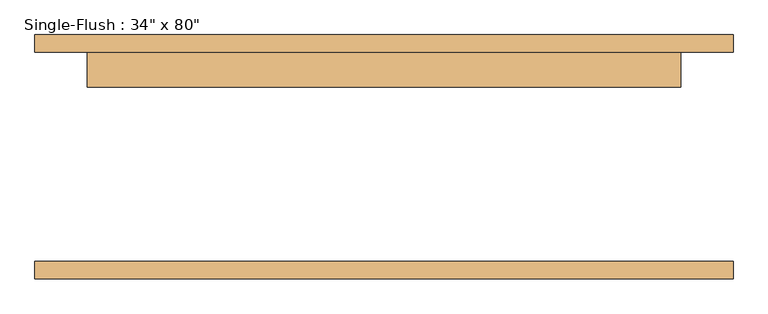
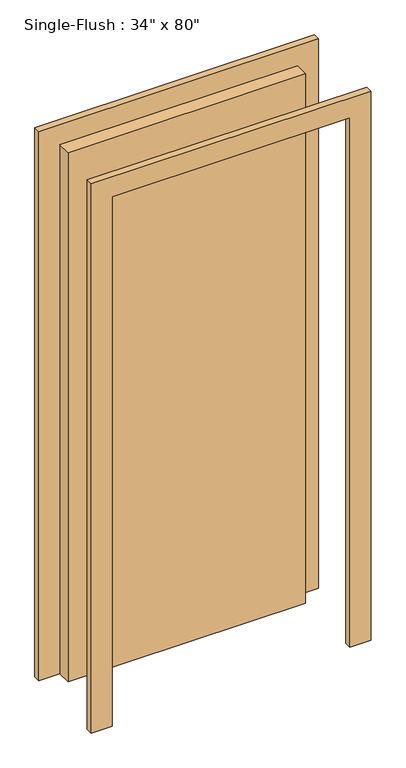
"""IFC4 building model written with IfcOpenShell, lengths in millimetres: door geometry."""

import ifcopenshell
import ifcopenshell.guid

model = None  # the IFC model being written
_history = None  # IfcOwnerHistory: only IFC2X3 demands one
_inside = {}  # id of a spatial element -> (the spatial element, [elements in it])
_under = {}  # id of a project, library or spatial element -> (it, [spatial elements below it])
_declared = {}  # id of a project -> (the project, [libraries it declares])
_typed = {}  # id of a type object -> (the type object, [elements of that type])
_made_of = {}  # id of a material, layer set ... -> (it, [elements and type objects made of it])


def new_model(schema):
    """Start an empty IFC model of exactly this schema.

    Asked for "IFC4X3", IfcOpenShell would pick the latest addendum, in which some entities
    have other attributes; the version numbers below select the first issue.
    IFC2X3 requires an IfcOwnerHistory on every rooted entity: one is made here for all.
    """
    global model, _history
    if schema == "IFC4X3":
        model = ifcopenshell.file(schema_version=(4, 3, 0, 0))
    else:
        model = ifcopenshell.file(schema=schema)
    _inside.clear()
    _under.clear()
    _declared.clear()
    _typed.clear()
    _made_of.clear()
    _history = None
    if model.schema == "IFC2X3":
        org = make("IfcOrganization", Name="unknown")
        user = make(
            "IfcPersonAndOrganization",
            ThePerson=make("IfcPerson", FamilyName="unknown"),
            TheOrganization=org,
        )
        app = make(
            "IfcApplication",
            ApplicationDeveloper=org,
            Version="unknown",
            ApplicationFullName="unknown",
            ApplicationIdentifier="unknown",
        )
        _history = make(
            "IfcOwnerHistory",
            OwningUser=user,
            OwningApplication=app,
            ChangeAction="ADDED",
            CreationDate=0,
        )
    return model


def make(cls, **values):
    """One entity of the class cls with the attributes given. An attribute that is None is left unset."""
    return model.create_entity(
        cls, **{name: value for name, value in values.items() if value is not None}
    )


def rooted(cls, **values):
    """An entity with a GlobalId (a new one), such as an element, a storey or a relation."""
    return make(cls, GlobalId=ifcopenshell.guid.new(), OwnerHistory=_history, **values)


def si_unit(unit_type, name, prefix=None):
    """IfcSIUnit, for example si_unit("LENGTHUNIT", "METRE", prefix="MILLI")."""
    return make("IfcSIUnit", UnitType=unit_type, Prefix=prefix, Name=name)


def assignment(units):
    """IfcUnitAssignment: the units of a project."""
    return None if units is None else make("IfcUnitAssignment", Units=units)


def point(xyz):
    """IfcCartesianPoint."""
    return None if xyz is None else make("IfcCartesianPoint", Coordinates=xyz)


def direction(xyz):
    """IfcDirection."""
    return None if xyz is None else make("IfcDirection", DirectionRatios=xyz)


def frame(location, z_axis=None, x_axis=None):
    """IfcAxis2Placement3D, a coordinate frame: its origin and axes. An axis left out is left unset."""
    return make(
        "IfcAxis2Placement3D",
        Location=point(location),
        Axis=direction(z_axis),
        RefDirection=direction(x_axis),
    )


def origin():
    """The frame at (0, 0, 0) with its axes left unset."""
    return frame((0.0, 0.0, 0.0))


def origin_with_axes():
    """The frame at (0, 0, 0) with the z axis (0, 0, 1) and the x axis (1, 0, 0) written out."""
    return frame((0.0, 0.0, 0.0), z_axis=(0.0, 0.0, 1.0), x_axis=(1.0, 0.0, 0.0))


def place(relative_to, where):
    """IfcLocalPlacement: puts the frame where relative to a parent placement (None: the world)."""
    return make(
        "IfcLocalPlacement", PlacementRelTo=relative_to, RelativePlacement=where
    )


def context(
    kind, dimensions, precision=None, world=None, true_north=None, identifier=None
):
    """IfcGeometricRepresentationContext, for example the 3D "Model" context."""
    return make(
        "IfcGeometricRepresentationContext",
        ContextIdentifier=identifier,
        ContextType=kind,
        CoordinateSpaceDimension=dimensions,
        Precision=precision,
        WorldCoordinateSystem=world,
        TrueNorth=true_north,
    )


def project(units=None, contexts=None):
    """IfcProject with its units and contexts."""
    return rooted(
        "IfcProject",
        Name="project",
        RepresentationContexts=contexts,
        UnitsInContext=assignment(units),
    )


def spatial(cls, under=None, at=None, **own):
    """A site, building, storey or space (cls), placed at a placement, below another one or the project."""
    s = rooted(cls, ObjectPlacement=at, **own)
    if under is not None:
        _under.setdefault(under.id(), (under, []))[1].append(s)
    return s


def polyline(points):
    """IfcPolyline through the points."""
    return make("IfcPolyline", Points=[point(p) for p in points])


def outline(outer, holes=None, kind="AREA"):
    """IfcArbitraryClosedProfileDef: a profile drawn as a closed curve; with holes, ...WithVoids."""
    if holes is None:
        return make("IfcArbitraryClosedProfileDef", ProfileType=kind, OuterCurve=outer)
    return make(
        "IfcArbitraryProfileDefWithVoids",
        ProfileType=kind,
        OuterCurve=outer,
        InnerCurves=holes,
    )


def extrude(swept, where, along, depth):
    """IfcExtrudedAreaSolid: the profile swept, set in the frame where, extruded along a direction by depth."""
    return make(
        "IfcExtrudedAreaSolid",
        SweptArea=swept,
        Position=where,
        ExtrudedDirection=direction(along),
        Depth=depth,
    )


def shape(context_of_items, identifier, shape_type, items):
    """IfcShapeRepresentation: the items that make up one representation, for example the "Body"."""
    return make(
        "IfcShapeRepresentation",
        ContextOfItems=context_of_items,
        RepresentationIdentifier=identifier,
        RepresentationType=shape_type,
        Items=items,
    )


def source(mapping_origin, context_of_items, identifier, shape_type, items):
    """IfcRepresentationMap: a shape defined once, which mapped items show again and again."""
    return make(
        "IfcRepresentationMap",
        MappingOrigin=mapping_origin,
        MappedRepresentation=shape(context_of_items, identifier, shape_type, items),
    )


def transform(
    local_origin,
    x_axis=None,
    y_axis=None,
    z_axis=None,
    scale=None,
    scale2=None,
    scale3=None,
    uniform=True,
):
    """IfcCartesianTransformationOperator3D, or its non-uniform kind. x_axis, y_axis, z_axis: its Axis1, 2, 3."""
    if uniform:
        return make(
            "IfcCartesianTransformationOperator3D",
            Axis1=direction(x_axis),
            Axis2=direction(y_axis),
            LocalOrigin=point(local_origin),
            Scale=scale,
            Axis3=direction(z_axis),
        )
    return make(
        "IfcCartesianTransformationOperator3DnonUniform",
        Axis1=direction(x_axis),
        Axis2=direction(y_axis),
        LocalOrigin=point(local_origin),
        Scale=scale,
        Axis3=direction(z_axis),
        Scale2=scale2,
        Scale3=scale3,
    )


def mapped(mapping_source, mapping_target):
    """IfcMappedItem: shows the shape of a source again, moved by a transform."""
    return make(
        "IfcMappedItem", MappingSource=mapping_source, MappingTarget=mapping_target
    )


def made_of(thing, what):
    """Note that an element or type object is made of a material, layer set ...; save() writes the relation."""
    if what is not None:
        _made_of.setdefault(what.id(), (what, []))[1].append(thing)
    return thing


def element(
    cls,
    number,
    at=None,
    inside=None,
    cuts=None,
    type_object=None,
    material=None,
    context=None,
    identifier="Body",
    shape_type=None,
    held_by="IfcProductDefinitionShape",
    body=None,
    shapes=None,
    **own,
):
    """One element of the class cls, such as IfcWall. Its Tag is "e" and its number.

    at: its placement. inside: the storey or other place that contains it. cuts: it is an
    opening in that element (IfcRelVoidsElement). A single representation is given by context,
    identifier, shape_type and body (its items); several are given by shapes. held_by: the class
    of the entity that holds the representations. save() writes the other relations.
    """
    e = rooted(cls, Tag="e%d" % number, ObjectPlacement=at, **own)
    if body is not None:
        shapes = [shape(context, identifier, shape_type, body)]
    if shapes is not None:
        e.Representation = make(held_by, Representations=shapes)
    if inside is not None:
        _inside.setdefault(inside.id(), (inside, []))[1].append(e)
    if cuts is not None:
        rooted(
            "IfcRelVoidsElement", RelatingBuildingElement=cuts, RelatedOpeningElement=e
        )
    if type_object is not None:
        _typed.setdefault(type_object.id(), (type_object, []))[1].append(e)
    return made_of(e, material)


def aggregate(whole, parts):
    """IfcRelAggregates: a whole, such as a stair, and the parts it consists of."""
    return rooted("IfcRelAggregates", RelatingObject=whole, RelatedObjects=parts)


def save(model, path):
    """Write the relations noted so far, then the file.

    IfcRelAggregates (storeys below a building ...), IfcRelContainedInSpatialStructure (elements
    in a storey), IfcRelDefinesByType, IfcRelAssociatesMaterial and IfcRelDeclares: one each for
    every whole, place, type object, material and project.
    """
    for whole, parts in _under.values():
        aggregate(whole, parts)
    for where, things in _inside.values():
        rooted(
            "IfcRelContainedInSpatialStructure",
            RelatedElements=things,
            RelatingStructure=where,
        )
    for kind, things in _typed.values():
        rooted("IfcRelDefinesByType", RelatedObjects=things, RelatingType=kind)
    for what, things in _made_of.values():
        rooted("IfcRelAssociatesMaterial", RelatedObjects=things, RelatingMaterial=what)
    for by, libraries in _declared.values():
        rooted("IfcRelDeclares", RelatingContext=by, RelatedDefinitions=libraries)
    model.write(path)


def door_93553381(model_context):
    return source(origin(), model_context, "Body", "SweptSolid", [
        extrude(outline(polyline([(2108.2, -508.0), (0.0, -508.0), (0.0, -431.8), (2032.0, -431.8), (2032.0, 431.8), (0.0, 431.8), (0.0, 508.0), (2108.2, 508.0), (2108.2, -508.0)])), frame((0.0, 152.4, 0.0), z_axis=(0.0, 1.0, 0.0), x_axis=(0.0, 0.0, 1.0)), (0.0, 0.0, 1.0), 25.4),
        extrude(outline(polyline([(2108.2, 508.0), (2108.2, -508.0), (0.0, -508.0), (0.0, -431.8), (2032.0, -431.8), (2032.0, 431.8), (0.0, 431.8), (0.0, 508.0), (2108.2, 508.0)])), frame((0.0, -177.8, 0.0), z_axis=(0.0, 1.0, 0.0), x_axis=(0.0, 0.0, 1.0)), (0.0, 0.0, 1.0), 25.4),
        extrude(outline(polyline([(431.8, 101.6), (-431.8, 101.6), (-431.8, 152.4), (431.8, 152.4), (431.8, 101.6)])), origin_with_axes(), (0.0, 0.0, 1.0), 2032.0),
    ])


if __name__ == "__main__":
    model = new_model("IFC4")
    model_context = context("Model", 3, world=origin())
    ifc_project = project(units=[si_unit("LENGTHUNIT", "METRE", prefix="MILLI")], contexts=[model_context])
    site = spatial("IfcSite", under=ifc_project)
    building = spatial("IfcBuilding", under=site)
    placement = place(None, origin())
    door_shape = door_93553381(model_context)
    element("IfcDoor", 1, ObjectType="Single-Flush : 34\" x 80\"", at=placement, inside=building, context=model_context, shape_type="MappedRepresentation", body=[
        mapped(door_shape, transform((0.0, 0.0, 0.0), x_axis=(1.0, 0.0, 0.0), y_axis=(0.0, 1.0, 0.0), z_axis=(0.0, 0.0, 1.0))),
    ])
    save(model, "model.ifc")

# Revit data of these elements
# Type "Single-Flush : 34\" x 80\""
#   Type Mark = "7"
#   Construction Type Id = "MDOOR"
#   Assembly Code = "C1020"
#   Analytic Construction = "Metal"
#   Thickness = 0' - 2"
#   Heat Transfer Coefficient (U) = 0.651978 BTU/(h·ft²·°F)
#   Height = 6' - 8"
#   Trim Projection Ext = 0' - 1"
#   Trim Projection Int = 0' - 1"
#   Trim Width = 0' - 3"
#   Width = 2' - 10"
#   Define Thermal Properties by = 1
#   Define Thermal Properties by = 1
#   Door Material = Door - Panel
#   Frame Material = Door - Frame
#   Visual Light Transmittance = 0
#   Solar Heat Gain Coefficient = 0
#   Function = (empty or 0)
#   Wall Closure = (empty or 0)
# Element 1 (IfcDoor, "Single-Flush : 34\" x 80\"")
#   Materials on its faces: "Door - Frame", "Door - Panel"
# Materials
#   "Door - Panel": class "Wood", colour RGB 210 159 95, transparency 0, Cost = 0
#   "Door - Frame": class "Miscellaneous", colour RGB 118 70 51, transparency 0, Cost = 0
